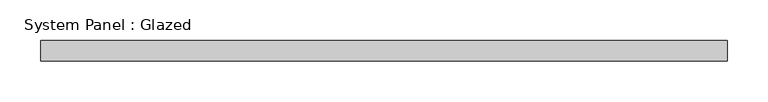
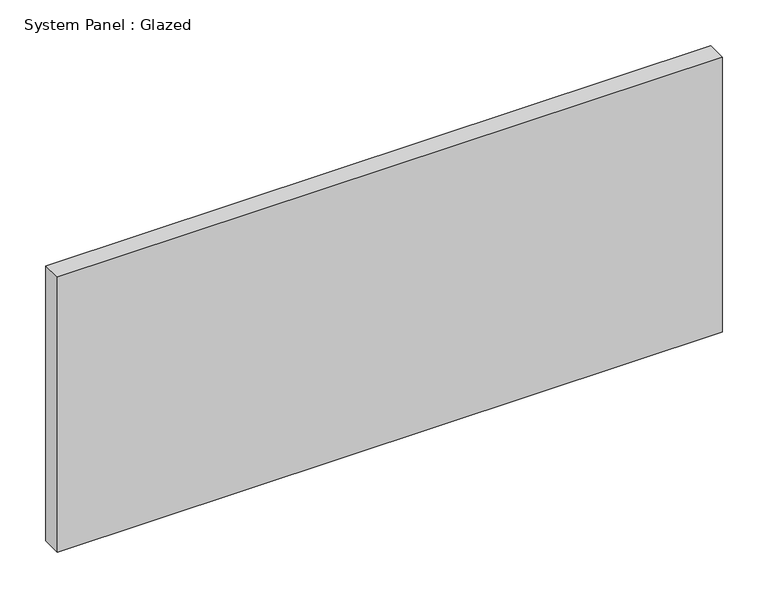
"""IFC4 building model written with IfcOpenShell, lengths in millimetres: plate geometry, System Panel : Glazed."""

from ifc_helpers import new_model, si_unit, origin, origin_with_axes, place, context, project, spatial, polyline, outline, extrude, source, transform, mapped, element, save


def system_panel_glazed_36114834(model_context):
    return source(origin(), model_context, "Body", "SweptSolid", [
        extrude(outline(polyline([(418.9393939, 24.5), (-418.9393939, 24.5), (-418.9393939, 49.5), (418.9393939, 49.5), (418.9393939, 24.5)])), origin_with_axes(), (0.0, 0.0, 1.0), 366.6666667),
    ])


if __name__ == "__main__":
    model = new_model("IFC4")
    model_context = context("Model", 3, world=origin())
    ifc_project = project(units=[si_unit("LENGTHUNIT", "METRE", prefix="MILLI")], contexts=[model_context])
    site = spatial("IfcSite", under=ifc_project)
    building = spatial("IfcBuilding", under=site)
    placement = place(None, origin())
    system_panel_glazed_shape = system_panel_glazed_36114834(model_context)
    element("IfcPlate", 1, ObjectType="System Panel : Glazed", at=placement, inside=building, context=model_context, shape_type="MappedRepresentation", body=[
        mapped(system_panel_glazed_shape, transform((0.0, 0.0, 0.0), x_axis=(1.0, 0.0, 0.0), y_axis=(0.0, 1.0, 0.0), z_axis=(0.0, 0.0, 1.0))),
    ])
    save(model, "model.ifc")

# Revit data of these elements
# Element 1 (IfcPlate, "System Panel : Glazed")
#   Materials on its faces: "Glass"
# Materials
#   "Glass": class "Glass", colour RGB 218 227 224, transparency 0.85, Description = "Soda Lime Glass", Cost = 0
